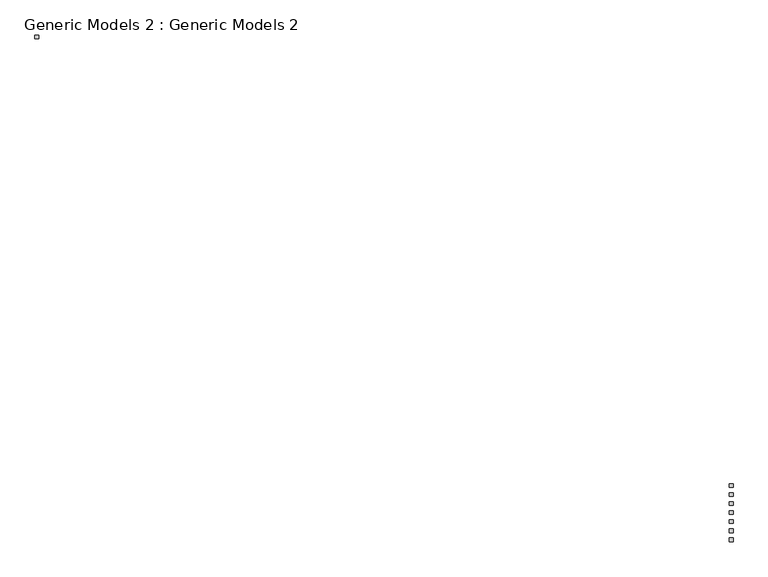
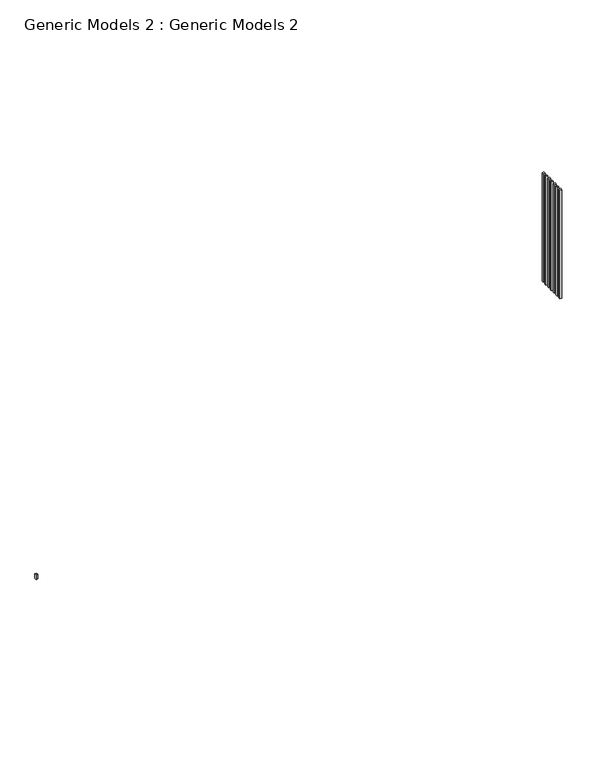
"""IFC4 building model written with IfcOpenShell, lengths in millimetres: proxy geometry, Generic Models 2 : Generic Models 2."""

from ifc_helpers import new_model, si_unit, frame, origin, origin_with_axes, place, context, project, spatial, polyline, outline, extrude, source, transform, mapped, element, save


def generic_models_2_generic_models_2_98282b11(model_context):
    return source(origin(), model_context, "Body", "SweptSolid", [
        extrude(outline(polyline([(16892.6280155, -2818.0630051), (16892.6280155, -2858.0630051), (16852.6280155, -2858.0630051), (16852.6280155, -2818.0630051), (16892.6280155, -2818.0630051)])), frame((0.0, 0.0, 6858.0), z_axis=(0.0, 0.0, 1.0), x_axis=(1.0, 0.0, 0.0)), (0.0, 0.0, 1.0), 2387.6),
        extrude(outline(polyline([(16892.6280155, -2918.0630051), (16892.6280155, -2958.0630051), (16852.6280155, -2958.0630051), (16852.6280155, -2918.0630051), (16892.6280155, -2918.0630051)])), frame((0.0, 0.0, 6858.0), z_axis=(0.0, 0.0, 1.0), x_axis=(1.0, 0.0, 0.0)), (0.0, 0.0, 1.0), 2387.6),
        extrude(outline(polyline([(16892.6280155, -3018.0630051), (16892.6280155, -3058.0630051), (16852.6280155, -3058.0630051), (16852.6280155, -3018.0630051), (16892.6280155, -3018.0630051)])), frame((0.0, 0.0, 6858.0), z_axis=(0.0, 0.0, 1.0), x_axis=(1.0, 0.0, 0.0)), (0.0, 0.0, 1.0), 2387.6),
        extrude(outline(polyline([(16892.6280155, -3118.0630051), (16892.6280155, -3158.0630051), (16852.6280155, -3158.0630051), (16852.6280155, -3118.0630051), (16892.6280155, -3118.0630051)])), frame((0.0, 0.0, 6858.0), z_axis=(0.0, 0.0, 1.0), x_axis=(1.0, 0.0, 0.0)), (0.0, 0.0, 1.0), 2387.6),
        extrude(outline(polyline([(16892.6280155, -3218.0630051), (16892.6280155, -3258.0630051), (16852.6280155, -3258.0630051), (16852.6280155, -3218.0630051), (16892.6280155, -3218.0630051)])), frame((0.0, 0.0, 6858.0), z_axis=(0.0, 0.0, 1.0), x_axis=(1.0, 0.0, 0.0)), (0.0, 0.0, 1.0), 2387.6),
        extrude(outline(polyline([(16892.6280155, -3318.0630051), (16892.6280155, -3358.0630051), (16852.6280155, -3358.0630051), (16852.6280155, -3318.0630051), (16892.6280155, -3318.0630051)])), frame((0.0, 0.0, 6858.0), z_axis=(0.0, 0.0, 1.0), x_axis=(1.0, 0.0, 0.0)), (0.0, 0.0, 1.0), 2387.6),
        extrude(outline(polyline([(16892.6280155, -3418.0630051), (16892.6280155, -3458.0630051), (16852.6280155, -3458.0630051), (16852.6280155, -3418.0630051), (16892.6280155, -3418.0630051)])), frame((0.0, 0.0, 6858.0), z_axis=(0.0, 0.0, 1.0), x_axis=(1.0, 0.0, 0.0)), (0.0, 0.0, 1.0), 2387.6),
        extrude(outline(polyline([(9215.8702604, 2147.6074866), (9215.8702604, 2107.6074866), (9175.8702604, 2107.6074866), (9175.8702604, 2147.6074866), (9215.8702604, 2147.6074866)])), origin_with_axes(), (0.0, 0.0, 1.0), 100.0),
    ])


if __name__ == "__main__":
    model = new_model("IFC4")
    model_context = context("Model", 3, world=origin())
    ifc_project = project(units=[si_unit("LENGTHUNIT", "METRE", prefix="MILLI")], contexts=[model_context])
    site = spatial("IfcSite", under=ifc_project)
    building = spatial("IfcBuilding", under=site)
    placement = place(None, origin())
    generic_models_2_generic_models_2_shape = generic_models_2_generic_models_2_98282b11(model_context)
    element("IfcBuildingElementProxy", 1, Name="Generic Models 2 : Generic Models 2", ObjectType="Generic Models 2 : Generic Models 2", at=placement, inside=building, context=model_context, shape_type="MappedRepresentation", body=[
        mapped(generic_models_2_generic_models_2_shape, transform((0.0, 0.0, 0.0), x_axis=(1.0, 0.0, 0.0), y_axis=(0.0, 1.0, 0.0), z_axis=(0.0, 0.0, 1.0))),
    ])
    save(model, "model.ifc")

# Revit data of these elements
# Element 1 (IfcBuildingElementProxy, "Generic Models 2 : Generic Models 2")
#   Materials on its faces: "MAT-1"
# Materials
#   "MAT-1": class "Generic", colour RGB 120 120 120, transparency 0, Cost = 0
